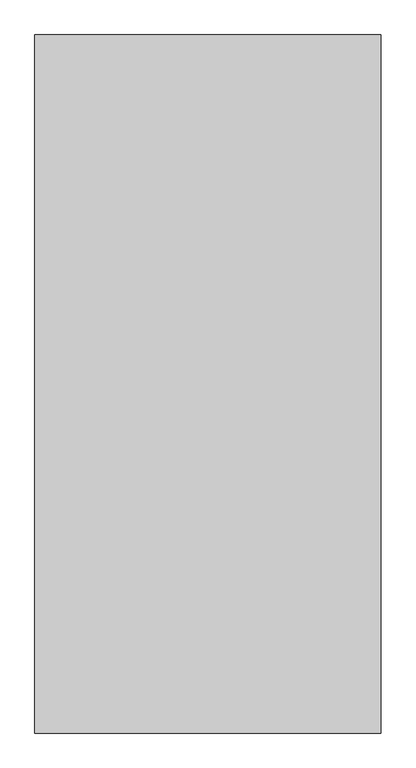
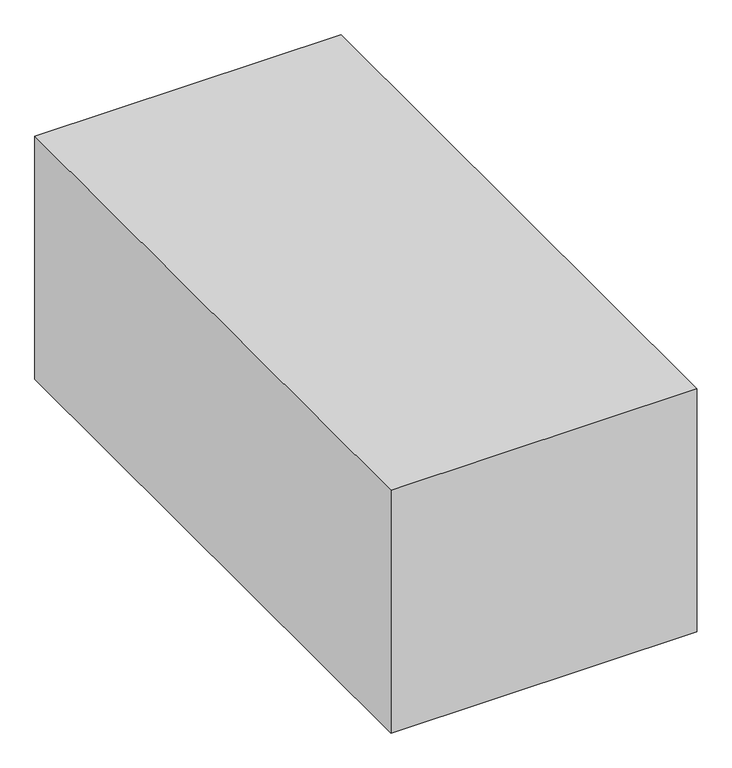
"""IFC4 building model written with IfcOpenShell, lengths in millimetres: proxy geometry, Space Planning Box_hec : Space Planning Box_hec."""

from ifc_helpers import new_model, si_unit, origin, origin_with_axes, place, context, project, spatial, polyline, outline, extrude, source, transform, mapped, element, save


def generic_models_f38cfd17(model_context):
    return source(origin(), model_context, "Body", "SweptSolid", [
        extrude(outline(polyline([(3100.0, 6250.0), (3100.0, -6250.0), (-3100.0, -6250.0), (-3100.0, 6250.0), (3100.0, 6250.0)])), origin_with_axes(), (0.0, 0.0, 1.0), 5200.0),
    ])


if __name__ == "__main__":
    model = new_model("IFC4")
    model_context = context("Model", 3, world=origin())
    ifc_project = project(units=[si_unit("LENGTHUNIT", "METRE", prefix="MILLI")], contexts=[model_context])
    site = spatial("IfcSite", under=ifc_project)
    building = spatial("IfcBuilding", under=site)
    placement = place(None, origin())
    generic_models_shape = generic_models_f38cfd17(model_context)
    element("IfcBuildingElementProxy", 1, Name="Space Planning Box_hec : Space Planning Box_hec", ObjectType="Space Planning Box_hec : Space Planning Box_hec", at=placement, inside=building, context=model_context, shape_type="MappedRepresentation", body=[
        mapped(generic_models_shape, transform((0.0, 0.0, 0.0), x_axis=(1.0, 0.0, 0.0), y_axis=(0.0, 1.0, 0.0), z_axis=(0.0, 0.0, 1.0))),
    ])
    save(model, "model.ifc")

# Revit data of these elements
# Type "Space Planning Box_hec : Space Planning Box_hec"
#   Type Comments = "..."
#   Room Name [instance default] = "?"
#   Interior Finish [instance default] = ""
#   Exterior Finish [instance default] = ""
#   Department [instance default] = ""
#   Assembly Code = "..."
#   ceiling height [instance default] = 0
#   Width [instance default] = 1524 mm
#   Program Area [instance default] = 0.00 m²
#   Length [instance default] = 1524 mm
#   Height [instance default] = 1524 mm
#   Area [instance default] = 2.32258 m²
#   Fill Color [instance default] = Cyan
#   Default Elevation = 0
# Element 1 (IfcBuildingElementProxy, "Space Planning Box_hec : Space Planning Box_hec")
#   Room Name = "Office-3"
#   Interior Finish = "IW1..N/A,,WB2..N/A,,FL6..N/A,,CL4..N/A"
#   Exterior Finish = "RF1..N/A,,EW1..N/A"
#   Department = "AR"
#   ceiling height = 2700
#   Width = 6200 mm
#   Program Area = 77.50 m²
#   Length = 12500 mm
#   Height = 5200 mm
#   Area = 77.50 m²
#   Materials on its faces: "Cyan"
# Materials
#   "Cyan": class "Generic", colour RGB 0 255 255, transparency 0.2, Cost = 0
